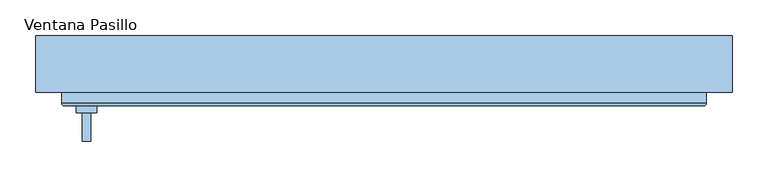
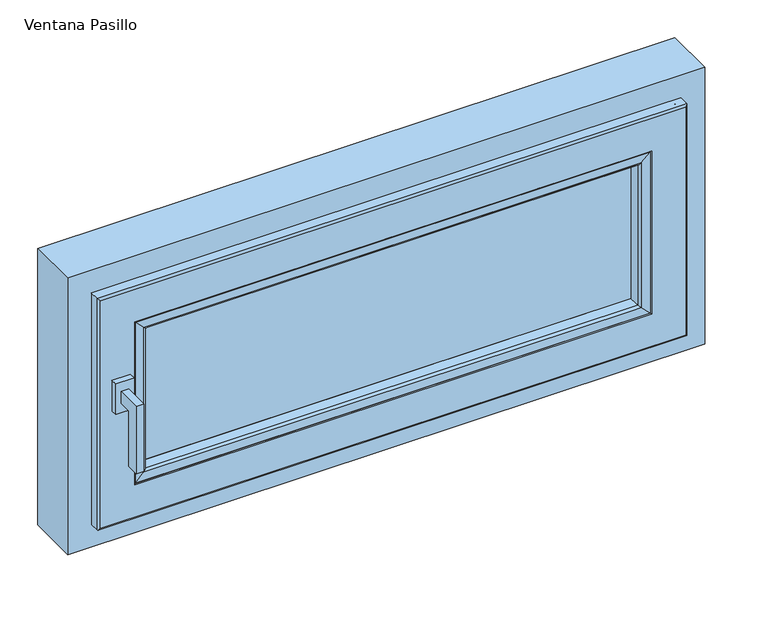
"""IFC4 building model written with IfcOpenShell, lengths in millimetres: window geometry, 2019_ES_Ventana_Replus_re80pvc301_10100_1-Hoja : Ventana Pasillo."""

import ifcopenshell
import ifcopenshell.guid

model = None  # the IFC model being written
_history = None  # IfcOwnerHistory: only IFC2X3 demands one
_inside = {}  # id of a spatial element -> (the spatial element, [elements in it])
_under = {}  # id of a project, library or spatial element -> (it, [spatial elements below it])
_declared = {}  # id of a project -> (the project, [libraries it declares])
_typed = {}  # id of a type object -> (the type object, [elements of that type])
_made_of = {}  # id of a material, layer set ... -> (it, [elements and type objects made of it])


def new_model(schema):
    """Start an empty IFC model of exactly this schema.

    Asked for "IFC4X3", IfcOpenShell would pick the latest addendum, in which some entities
    have other attributes; the version numbers below select the first issue.
    IFC2X3 requires an IfcOwnerHistory on every rooted entity: one is made here for all.
    """
    global model, _history
    if schema == "IFC4X3":
        model = ifcopenshell.file(schema_version=(4, 3, 0, 0))
    else:
        model = ifcopenshell.file(schema=schema)
    _inside.clear()
    _under.clear()
    _declared.clear()
    _typed.clear()
    _made_of.clear()
    _history = None
    if model.schema == "IFC2X3":
        org = make("IfcOrganization", Name="unknown")
        user = make(
            "IfcPersonAndOrganization",
            ThePerson=make("IfcPerson", FamilyName="unknown"),
            TheOrganization=org,
        )
        app = make(
            "IfcApplication",
            ApplicationDeveloper=org,
            Version="unknown",
            ApplicationFullName="unknown",
            ApplicationIdentifier="unknown",
        )
        _history = make(
            "IfcOwnerHistory",
            OwningUser=user,
            OwningApplication=app,
            ChangeAction="ADDED",
            CreationDate=0,
        )
    return model


def make(cls, **values):
    """One entity of the class cls with the attributes given. An attribute that is None is left unset."""
    return model.create_entity(
        cls, **{name: value for name, value in values.items() if value is not None}
    )


def rooted(cls, **values):
    """An entity with a GlobalId (a new one), such as an element, a storey or a relation."""
    return make(cls, GlobalId=ifcopenshell.guid.new(), OwnerHistory=_history, **values)


def si_unit(unit_type, name, prefix=None):
    """IfcSIUnit, for example si_unit("LENGTHUNIT", "METRE", prefix="MILLI")."""
    return make("IfcSIUnit", UnitType=unit_type, Prefix=prefix, Name=name)


def assignment(units):
    """IfcUnitAssignment: the units of a project."""
    return None if units is None else make("IfcUnitAssignment", Units=units)


def point(xyz):
    """IfcCartesianPoint."""
    return None if xyz is None else make("IfcCartesianPoint", Coordinates=xyz)


def direction(xyz):
    """IfcDirection."""
    return None if xyz is None else make("IfcDirection", DirectionRatios=xyz)


def frame(location, z_axis=None, x_axis=None):
    """IfcAxis2Placement3D, a coordinate frame: its origin and axes. An axis left out is left unset."""
    return make(
        "IfcAxis2Placement3D",
        Location=point(location),
        Axis=direction(z_axis),
        RefDirection=direction(x_axis),
    )


def origin():
    """The frame at (0, 0, 0) with its axes left unset."""
    return frame((0.0, 0.0, 0.0))


def place(relative_to, where):
    """IfcLocalPlacement: puts the frame where relative to a parent placement (None: the world)."""
    return make(
        "IfcLocalPlacement", PlacementRelTo=relative_to, RelativePlacement=where
    )


def context(
    kind, dimensions, precision=None, world=None, true_north=None, identifier=None
):
    """IfcGeometricRepresentationContext, for example the 3D "Model" context."""
    return make(
        "IfcGeometricRepresentationContext",
        ContextIdentifier=identifier,
        ContextType=kind,
        CoordinateSpaceDimension=dimensions,
        Precision=precision,
        WorldCoordinateSystem=world,
        TrueNorth=true_north,
    )


def project(units=None, contexts=None):
    """IfcProject with its units and contexts."""
    return rooted(
        "IfcProject",
        Name="project",
        RepresentationContexts=contexts,
        UnitsInContext=assignment(units),
    )


def spatial(cls, under=None, at=None, **own):
    """A site, building, storey or space (cls), placed at a placement, below another one or the project."""
    s = rooted(cls, ObjectPlacement=at, **own)
    if under is not None:
        _under.setdefault(under.id(), (under, []))[1].append(s)
    return s


def polyline(points):
    """IfcPolyline through the points."""
    return make("IfcPolyline", Points=[point(p) for p in points])


def ellipse_curve(where, semi_axis1, semi_axis2):
    """IfcEllipse in the frame where."""
    return make(
        "IfcEllipse", Position=where, SemiAxis1=semi_axis1, SemiAxis2=semi_axis2
    )


def outline(outer, holes=None, kind="AREA"):
    """IfcArbitraryClosedProfileDef: a profile drawn as a closed curve; with holes, ...WithVoids."""
    if holes is None:
        return make("IfcArbitraryClosedProfileDef", ProfileType=kind, OuterCurve=outer)
    return make(
        "IfcArbitraryProfileDefWithVoids",
        ProfileType=kind,
        OuterCurve=outer,
        InnerCurves=holes,
    )


def extrude(swept, where, along, depth):
    """IfcExtrudedAreaSolid: the profile swept, set in the frame where, extruded along a direction by depth."""
    return make(
        "IfcExtrudedAreaSolid",
        SweptArea=swept,
        Position=where,
        ExtrudedDirection=direction(along),
        Depth=depth,
    )


def shape(context_of_items, identifier, shape_type, items):
    """IfcShapeRepresentation: the items that make up one representation, for example the "Body"."""
    return make(
        "IfcShapeRepresentation",
        ContextOfItems=context_of_items,
        RepresentationIdentifier=identifier,
        RepresentationType=shape_type,
        Items=items,
    )


def source(mapping_origin, context_of_items, identifier, shape_type, items):
    """IfcRepresentationMap: a shape defined once, which mapped items show again and again."""
    return make(
        "IfcRepresentationMap",
        MappingOrigin=mapping_origin,
        MappedRepresentation=shape(context_of_items, identifier, shape_type, items),
    )


def transform(
    local_origin,
    x_axis=None,
    y_axis=None,
    z_axis=None,
    scale=None,
    scale2=None,
    scale3=None,
    uniform=True,
):
    """IfcCartesianTransformationOperator3D, or its non-uniform kind. x_axis, y_axis, z_axis: its Axis1, 2, 3."""
    if uniform:
        return make(
            "IfcCartesianTransformationOperator3D",
            Axis1=direction(x_axis),
            Axis2=direction(y_axis),
            LocalOrigin=point(local_origin),
            Scale=scale,
            Axis3=direction(z_axis),
        )
    return make(
        "IfcCartesianTransformationOperator3DnonUniform",
        Axis1=direction(x_axis),
        Axis2=direction(y_axis),
        LocalOrigin=point(local_origin),
        Scale=scale,
        Axis3=direction(z_axis),
        Scale2=scale2,
        Scale3=scale3,
    )


def mapped(mapping_source, mapping_target):
    """IfcMappedItem: shows the shape of a source again, moved by a transform."""
    return make(
        "IfcMappedItem", MappingSource=mapping_source, MappingTarget=mapping_target
    )


def made_of(thing, what):
    """Note that an element or type object is made of a material, layer set ...; save() writes the relation."""
    if what is not None:
        _made_of.setdefault(what.id(), (what, []))[1].append(thing)
    return thing


def element(
    cls,
    number,
    at=None,
    inside=None,
    cuts=None,
    type_object=None,
    material=None,
    context=None,
    identifier="Body",
    shape_type=None,
    held_by="IfcProductDefinitionShape",
    body=None,
    shapes=None,
    **own,
):
    """One element of the class cls, such as IfcWall. Its Tag is "e" and its number.

    at: its placement. inside: the storey or other place that contains it. cuts: it is an
    opening in that element (IfcRelVoidsElement). A single representation is given by context,
    identifier, shape_type and body (its items); several are given by shapes. held_by: the class
    of the entity that holds the representations. save() writes the other relations.
    """
    e = rooted(cls, Tag="e%d" % number, ObjectPlacement=at, **own)
    if body is not None:
        shapes = [shape(context, identifier, shape_type, body)]
    if shapes is not None:
        e.Representation = make(held_by, Representations=shapes)
    if inside is not None:
        _inside.setdefault(inside.id(), (inside, []))[1].append(e)
    if cuts is not None:
        rooted(
            "IfcRelVoidsElement", RelatingBuildingElement=cuts, RelatedOpeningElement=e
        )
    if type_object is not None:
        _typed.setdefault(type_object.id(), (type_object, []))[1].append(e)
    return made_of(e, material)


def aggregate(whole, parts):
    """IfcRelAggregates: a whole, such as a stair, and the parts it consists of."""
    return rooted("IfcRelAggregates", RelatingObject=whole, RelatedObjects=parts)


def save(model, path):
    """Write the relations noted so far, then the file.

    IfcRelAggregates (storeys below a building ...), IfcRelContainedInSpatialStructure (elements
    in a storey), IfcRelDefinesByType, IfcRelAssociatesMaterial and IfcRelDeclares: one each for
    every whole, place, type object, material and project.
    """
    for whole, parts in _under.values():
        aggregate(whole, parts)
    for where, things in _inside.values():
        rooted(
            "IfcRelContainedInSpatialStructure",
            RelatedElements=things,
            RelatingStructure=where,
        )
    for kind, things in _typed.values():
        rooted("IfcRelDefinesByType", RelatedObjects=things, RelatingType=kind)
    for what, things in _made_of.values():
        rooted("IfcRelAssociatesMaterial", RelatedObjects=things, RelatingMaterial=what)
    for by, libraries in _declared.values():
        rooted("IfcRelDeclares", RelatingContext=by, RelatedDefinitions=libraries)
    model.write(path)


def plane_surface(at):
    """IfcPlane: the flat surface through the origin of the frame at, square to its z axis."""
    return make("IfcPlane", Position=at)


def cylinder_surface(at, radius):
    """IfcCylindricalSurface: all points at the distance radius from the z axis of the frame at."""
    return make("IfcCylindricalSurface", Position=at, Radius=radius)


def advanced_brep(points, edges, surfaces, faces):
    """IfcAdvancedBrep: a solid bounded by faces that lie on surfaces and meet in shared edges.

    An edge is (start, end): straight between two places in points (the first is 0);
    or (start, end, curve); or (start, end, curve, False) where it runs against its curve.
    A face is (place in surfaces, loops), or (place, loops, False) where it looks against
    its surface's normal. A loop lists edges by number (the first is 1), with a minus sign
    where the edge is run from its end to its start. The first loop is the outer one.
    """
    corners = [point(p) for p in points]
    vertices = [make("IfcVertexPoint", VertexGeometry=c) for c in corners]
    made = []
    for start, end, *more in edges:
        made.append(
            make(
                "IfcEdgeCurve",
                EdgeStart=vertices[start],
                EdgeEnd=vertices[end],
                EdgeGeometry=more[0] if more else make("IfcPolyline", Points=[corners[start], corners[end]]),
                SameSense=more[1] if len(more) > 1 else True,
            )
        )
    hull = []
    for where, loops, *sense in faces:
        bounds = []
        for j, loop in enumerate(loops):
            ring = [make("IfcOrientedEdge", EdgeElement=made[abs(k) - 1], Orientation=k > 0) for k in loop]
            bounds.append(
                make(
                    "IfcFaceOuterBound" if j == 0 else "IfcFaceBound",
                    Bound=make("IfcEdgeLoop", EdgeList=ring),
                    Orientation=True,
                )
            )
        hull.append(make("IfcAdvancedFace", Bounds=bounds, FaceSurface=surfaces[where], SameSense=sense[0] if sense else True))
    return make("IfcAdvancedBrep", Outer=make("IfcClosedShell", CfsFaces=hull))


def ventana_pasillo_7f72e0b0(model_context):
    return source(origin(), model_context, "Body", "SolidModel", [
        extrude(outline(polyline([(-78.4999991, 1070.0), (-78.4999991, 1050.0), (-98.4999991, 1050.0), (-98.4999991, 960.0), (-118.4999991, 960.0), (-118.4999991, 1070.0), (-78.4999991, 1070.0)])), frame((-424.1999993, 0.0, 0.0), z_axis=(1.0, 0.0, 0.0), x_axis=(0.0, 1.0, 0.0)), (0.0, 0.0, 1.0), 12.0),
        extrude(outline(polyline([(-403.9687607, -78.4999991), (-432.4312378, -78.4999991), (-432.4312378, -68.4999991), (-403.9687607, -68.4999991), (-403.9687607, -78.4999991)])), frame((0.0, 0.0, 1035.217127), z_axis=(0.0, 0.0, 1.0), x_axis=(1.0, 0.0, 0.0)), (0.0, 0.0, 1.0), 49.565746),
        extrude(outline(polyline([(1157.2, 387.1999993), (1157.2, -387.1999993), (909.8, -387.1999993), (909.8, 387.1999993), (1157.2, 387.1999993)]), holes=[polyline([(917.8, 379.1999993), (917.8, -379.1999993), (1149.2, -379.1999993), (1149.2, 379.1999993), (917.8, 379.1999993)])]), frame((0.0, -26.9999999, 0.0), z_axis=(0.0, 1.0, 0.0), x_axis=(0.0, 0.0, 1.0)), (0.0, 0.0, 1.0), 16.0),
        extrude(outline(polyline([(1157.1868066, 387.1868058), (1157.1868066, -387.1868058), (909.8131934, -387.1868058), (909.8131934, 387.1868058), (1157.1868066, 387.1868058)]), holes=[polyline([(917.8, 379.1999993), (917.8, -379.1999993), (1149.2, -379.1999993), (1149.2, 379.1999993), (917.8, 379.1999993)])]), frame((0.0, -47.0000001, 0.0), z_axis=(0.0, 1.0, 0.0), x_axis=(0.0, 0.0, 1.0)), (0.0, 0.0, 1.0), 16.0),
        extrude(outline(polyline([(387.1999993, -6.9999997), (387.1999993, -10.9999999), (-387.1999993, -10.9999999), (-387.1999993, -6.9999997), (387.1999993, -6.9999997)])), frame((0.0, 0.0, 903.7946451), z_axis=(0.0, 0.0, 1.0), x_axis=(1.0, 0.0, 0.0)), (0.0, 0.0, 1.0), 259.4053549),
        extrude(outline(polyline([(387.1999993, -26.9999999), (387.1999993, -31.0000001), (-387.1999993, -31.0000001), (-387.1999993, -26.9999999), (387.1999993, -26.9999999)])), frame((0.0, 0.0, 903.7946451), z_axis=(0.0, 0.0, 1.0), x_axis=(1.0, 0.0, 0.0)), (0.0, 0.0, 1.0), 259.4053549),
        extrude(outline(polyline([(387.1999993, -47.0000001), (387.1999993, -51.0000003), (-387.1999993, -51.0000003), (-387.1999993, -47.0000001), (387.1999993, -47.0000001)])), frame((0.0, 0.0, 903.7946451), z_axis=(0.0, 0.0, 1.0), x_axis=(1.0, 0.0, 0.0)), (0.0, 0.0, 1.0), 259.4053549),
        advanced_brep(
        [(377.2913171, 9.2764571, 1147.2913178), (380.1890946, 11.5, 1150.1890953), (380.1890946, 11.5, 919.8109047), (377.2913171, 9.2764571, 922.7086822), (420.1999993, 11.5, 879.8), (-420.1999993, 11.5, 879.8), (-420.1999993, 11.5, 1190.2), (420.1999993, 11.5, 1190.2), (-380.1890946, 11.5, 1150.1890953), (-380.1890946, 11.5, 919.8109047), (-377.2913171, 9.2764571, 922.7086822), (374.1757968, -2.3508228, 1144.1757976), (374.1757968, -2.3508228, 925.8242024), (-374.1757968, -2.3508228, 925.8242024), (374.6739305, -3.0000033, 1144.6739313), (374.6739305, -3.0000033, 925.3260687), (-374.6739305, -3.0000033, 925.3260687), (381.1999993, -3.0000033, 1151.2), (-381.1999993, -3.0000033, 1151.2), (-381.1999993, -3.0000033, 918.8), (381.1999993, -3.0000033, 918.8), (-374.6739305, -3.0000033, 1144.6739313), (381.1999993, -6.9999997, 1151.2), (381.1999993, -6.9999997, 918.8), (-381.1999993, -6.9999997, 918.8), (401.8162192, -6.9999997, 1171.8162199), (-401.8162192, -6.9999997, 1171.8162199), (-401.8162192, -6.9999997, 898.1837801), (401.8162192, -6.9999997, 898.1837801), (-381.1999993, -6.9999997, 1151.2), (399.1999993, -25.6153717, 1169.2), (399.1999993, -25.6153717, 900.8), (-399.1999993, -25.6153717, 900.8), (399.1999993, -56.4999995, 1169.2), (399.1999993, -56.4999995, 900.8), (-399.1999993, -56.4999995, 900.8), (-399.1999993, -56.4999995, 1169.2), (387.1999993, -56.4999995, 1157.2), (-387.1999993, -56.4999995, 1157.2), (-387.1999993, -56.4999995, 912.8), (387.1999993, -56.4999995, 912.8), (387.1999993, -51.0000003, 1157.2), (387.1999993, -51.0000003, 912.8), (-387.1999993, -51.0000003, 912.8), (-387.1999993, -51.0000003, 1157.2), (376.007687, -51.0000003, 1146.0076877), (-376.007687, -51.0000003, 1146.0076877), (-376.007687, -51.0000003, 923.9923123), (376.007687, -51.0000003, 923.9923123), (375.4940999, -51.6693201, 1145.4941006), (375.4940999, -51.6693201, 924.5058994), (-375.4940999, -51.6693201, 924.5058994), (378.8993918, -64.3780426, 1148.8993925), (378.8993918, -64.3780426, 921.1006075), (-378.8993918, -64.3780426, 921.1006075), (382.6234971, -67.3403297, 1152.6234978), (382.6234971, -67.3403297, 917.3765022), (-382.6234971, -67.3403297, 917.3765022), (395.6488427, -67.7951848, 1165.6488434), (395.6488427, -67.7951848, 904.3511566), (-395.6488427, -67.7951848, 904.3511566), (396.1999993, -67.2629391, 1166.2), (396.1999993, -67.2629391, 903.8), (-396.1999993, -67.2629391, 903.8), (397.4370593, -68.4999991, 1167.43706), (397.4370593, -68.4999991, 902.56294), (-397.4370593, -68.4999991, 902.56294), (450.1999993, -68.4999991, 1220.2), (-450.1999993, -68.4999991, 1220.2), (-450.1999993, -68.4999991, 849.8), (450.1999993, -68.4999991, 849.8), (-397.4370593, -68.4999991, 1167.43706), (453.1999993, -65.4999991, 1223.2), (453.1999993, -65.4999991, 846.8), (-453.1999993, -65.4999991, 846.8), (453.1999993, -50.0, 1223.2), (453.1999993, -50.0, 846.8), (-453.1999993, -50.0, 846.8), (-453.1999993, -50.0, 1223.2), (433.1999993, -50.0, 1203.2), (-433.1999993, -50.0, 1203.2), (-433.1999993, -50.0, 866.8), (433.1999993, -50.0, 866.8), (433.1999993, -11.9999991, 866.8), (433.1999993, -11.9999991, 1203.2), (-433.1999993, -11.9999991, 866.8), (-433.1999993, -11.9999991, 1203.2), (420.1999993, -11.9999991, 1190.2), (-420.1999993, -11.9999991, 1190.2), (-420.1999993, -11.9999991, 879.8), (420.1999993, -11.9999991, 879.8), (-377.2913171, 9.2764571, 1147.2913178), (-374.1757968, -2.3508228, 1144.1757976), (-399.1999993, -25.6153717, 1169.2), (-375.4940999, -51.6693201, 1145.4941006), (-378.8993918, -64.3780426, 1148.8993925), (-382.6234971, -67.3403297, 1152.6234978), (-395.6488427, -67.7951848, 1165.6488434), (-396.1999993, -67.2629391, 1166.2), (-453.1999993, -65.4999991, 1223.2)],
        [
            (0, 1, ellipse_curve(frame((380.1890946, 8.5, 1150.1890953), z_axis=(0.7071067811865475, 0.0, -0.7071067811865475), x_axis=(0.7071067811865474, 0.0, 0.7071067811865476)), 4.2426407, 3.0)),
            (1, 2),
            (2, 3, ellipse_curve(frame((380.1890946, 8.5, 919.8109047), z_axis=(0.7071067811865475, 0.0, 0.7071067811865475), x_axis=(-0.7071067811865474, 0.0, 0.7071067811865476)), 4.2426407, 3.0)),
            (3, 0),
            (4, 5),
            (5, 6),
            (6, 7),
            (7, 4),
            (1, 8),
            (8, 9),
            (9, 2),
            (9, 10, ellipse_curve(frame((-380.1890946, 8.5, 919.8109047), z_axis=(0.7071067811865475, 0.0, -0.7071067811865475), x_axis=(0.7071067811865476, 0.0, 0.7071067811865474)), 4.2426407, 3.0)),
            (10, 3),
            (11, 0),
            (3, 12),
            (12, 11),
            (10, 13),
            (13, 12),
            (14, 11, ellipse_curve(frame((374.6739305, -2.4842973, 1144.6739313), z_axis=(0.7071067811865475, 0.0, -0.7071067811865475), x_axis=(0.7071067811865474, 0.0, 0.7071067811865476)), 0.7293184, 0.515706)),
            (12, 15, ellipse_curve(frame((374.6739305, -2.4842973, 925.3260687), z_axis=(0.7071067811865475, 0.0, 0.7071067811865475), x_axis=(-0.7071067811865474, 0.0, 0.7071067811865476)), 0.7293184, 0.515706)),
            (15, 14),
            (13, 16, ellipse_curve(frame((-374.6739305, -2.4842973, 925.3260687), z_axis=(0.7071067811865475, 0.0, -0.7071067811865475), x_axis=(0.7071067811865476, 0.0, 0.7071067811865474)), 0.7293184, 0.515706)),
            (16, 15),
            (17, 18),
            (18, 19),
            (19, 20),
            (20, 17),
            (16, 21),
            (21, 14),
            (22, 17),
            (20, 23),
            (23, 22),
            (19, 24),
            (24, 23),
            (25, 26),
            (26, 27),
            (27, 28),
            (28, 25),
            (24, 29),
            (29, 22),
            (30, 25),
            (28, 31),
            (31, 30),
            (27, 32),
            (32, 31),
            (33, 30),
            (31, 34),
            (34, 33),
            (32, 35),
            (35, 34),
            (35, 36),
            (36, 33),
            (37, 38),
            (38, 39),
            (39, 40),
            (40, 37),
            (41, 37),
            (40, 42),
            (42, 41),
            (39, 43),
            (43, 42),
            (43, 44),
            (44, 41),
            (45, 46),
            (46, 47),
            (47, 48),
            (48, 45),
            (49, 45, ellipse_curve(frame((376.007687, -51.5317048, 1146.0076877), z_axis=(0.7071067811865475, 0.0, -0.7071067811865475), x_axis=(0.7071067811865474, 0.0, 0.7071067811865476)), 0.7519437, 0.5317045)),
            (48, 50, ellipse_curve(frame((376.007687, -51.5317048, 923.9923123), z_axis=(0.7071067811865475, 0.0, 0.7071067811865475), x_axis=(-0.7071067811865474, 0.0, 0.7071067811865476)), 0.7519437, 0.5317045)),
            (50, 49),
            (47, 51, ellipse_curve(frame((-376.007687, -51.5317048, 923.9923123), z_axis=(0.7071067811865475, 0.0, -0.7071067811865475), x_axis=(0.7071067811865476, 0.0, 0.7071067811865474)), 0.7519437, 0.5317045)),
            (51, 50),
            (52, 49),
            (50, 53),
            (53, 52),
            (51, 54),
            (54, 53),
            (55, 52, ellipse_curve(frame((382.7630951, -63.3427664, 1152.7630958), z_axis=(0.7071067811865475, 0.0, -0.7071067811865475), x_axis=(0.7071067811865474, 0.0, 0.7071067811865476)), 5.6568542, 4.0)),
            (53, 56, ellipse_curve(frame((382.7630951, -63.3427664, 917.2369042), z_axis=(0.7071067811865475, 0.0, 0.7071067811865475), x_axis=(-0.7071067811865474, 0.0, 0.7071067811865476)), 5.6568542, 4.0)),
            (56, 55),
            (54, 57, ellipse_curve(frame((-382.7630951, -63.3427664, 917.2369042), z_axis=(0.7071067811865475, 0.0, -0.7071067811865475), x_axis=(0.7071067811865476, 0.0, 0.7071067811865474)), 5.6568542, 4.0)),
            (57, 56),
            (58, 55),
            (56, 59),
            (59, 58),
            (57, 60),
            (60, 59),
            (61, 58, ellipse_curve(frame((395.6674291, -67.2629391, 1165.6674299), z_axis=(0.7071067811865475, 0.0, -0.7071067811865475), x_axis=(0.7071067811865474, 0.0, 0.7071067811865476)), 0.7531679, 0.5325701)),
            (59, 62, ellipse_curve(frame((395.6674291, -67.2629391, 904.3325701), z_axis=(0.7071067811865475, 0.0, 0.7071067811865475), x_axis=(-0.7071067811865474, 0.0, 0.7071067811865476)), 0.7531679, 0.5325701)),
            (62, 61),
            (60, 63, ellipse_curve(frame((-395.6674291, -67.2629391, 904.3325701), z_axis=(0.7071067811865475, 0.0, -0.7071067811865475), x_axis=(0.7071067811865476, 0.0, 0.7071067811865474)), 0.7531679, 0.5325701)),
            (63, 62),
            (64, 61, ellipse_curve(frame((397.4370593, -67.2629391, 1167.43706), z_axis=(0.7071067811865475, 0.0, -0.7071067811865475), x_axis=(0.7071067811865474, 0.0, 0.7071067811865476)), 1.7494671, 1.23706)),
            (62, 65, ellipse_curve(frame((397.4370593, -67.2629391, 902.56294), z_axis=(0.7071067811865475, 0.0, 0.7071067811865475), x_axis=(-0.7071067811865474, 0.0, 0.7071067811865476)), 1.7494671, 1.23706)),
            (65, 64),
            (63, 66, ellipse_curve(frame((-397.4370593, -67.2629391, 902.56294), z_axis=(0.7071067811865475, 0.0, -0.7071067811865475), x_axis=(0.7071067811865476, 0.0, 0.7071067811865474)), 1.7494671, 1.23706)),
            (66, 65),
            (67, 68),
            (68, 69),
            (69, 70),
            (70, 67),
            (66, 71),
            (71, 64),
            (72, 67, ellipse_curve(frame((450.1999993, -65.4999991, 1220.2), z_axis=(0.7071067811865475, 0.0, -0.7071067811865475), x_axis=(0.7071067811865474, 0.0, 0.7071067811865476)), 4.2426407, 3.0)),
            (70, 73, ellipse_curve(frame((450.1999993, -65.4999991, 849.8), z_axis=(0.7071067811865475, 0.0, 0.7071067811865475), x_axis=(-0.7071067811865474, 0.0, 0.7071067811865476)), 4.2426407, 3.0)),
            (73, 72),
            (69, 74, ellipse_curve(frame((-450.1999993, -65.4999991, 849.8), z_axis=(0.7071067811865475, 0.0, -0.7071067811865475), x_axis=(0.7071067811865476, 0.0, 0.7071067811865474)), 4.2426407, 3.0)),
            (74, 73),
            (75, 72),
            (73, 76),
            (76, 75),
            (74, 77),
            (77, 76),
            (77, 78),
            (78, 75),
            (79, 80),
            (80, 81),
            (81, 82),
            (82, 79),
            (82, 83),
            (83, 84),
            (84, 79),
            (81, 85),
            (85, 83),
            (85, 86),
            (86, 84),
            (87, 88),
            (88, 89),
            (89, 90),
            (90, 87),
            (90, 4),
            (7, 87),
            (89, 5),
            (8, 91, ellipse_curve(frame((-380.1890946, 8.5, 1150.1890953), z_axis=(-0.7071067811865475, 0.0, -0.7071067811865475), x_axis=(0.7071067811865474, 0.0, -0.7071067811865476)), 4.2426407, 3.0)),
            (91, 10),
            (91, 92),
            (92, 13),
            (92, 21, ellipse_curve(frame((-374.6739305, -2.4842973, 1144.6739313), z_axis=(-0.7071067811865475, 0.0, -0.7071067811865475), x_axis=(0.7071067811865474, 0.0, -0.7071067811865476)), 0.7293184, 0.515706)),
            (18, 29),
            (26, 93),
            (93, 32),
            (93, 36),
            (38, 44),
            (46, 94, ellipse_curve(frame((-376.007687, -51.5317048, 1146.0076877), z_axis=(-0.7071067811865475, 0.0, -0.7071067811865475), x_axis=(0.7071067811865474, 0.0, -0.7071067811865476)), 0.7519437, 0.5317045)),
            (94, 51),
            (94, 95),
            (95, 54),
            (95, 96, ellipse_curve(frame((-382.7630951, -63.3427664, 1152.7630958), z_axis=(-0.7071067811865475, 0.0, -0.7071067811865475), x_axis=(0.7071067811865474, 0.0, -0.7071067811865476)), 5.6568542, 4.0)),
            (96, 57),
            (96, 97),
            (97, 60),
            (97, 98, ellipse_curve(frame((-395.6674291, -67.2629391, 1165.6674299), z_axis=(-0.7071067811865475, 0.0, -0.7071067811865475), x_axis=(0.7071067811865474, 0.0, -0.7071067811865476)), 0.7531679, 0.5325701)),
            (98, 63),
            (98, 71, ellipse_curve(frame((-397.4370593, -67.2629391, 1167.43706), z_axis=(-0.7071067811865475, 0.0, -0.7071067811865475), x_axis=(0.7071067811865474, 0.0, -0.7071067811865476)), 1.7494671, 1.23706)),
            (68, 99, ellipse_curve(frame((-450.1999993, -65.4999991, 1220.2), z_axis=(-0.7071067811865475, 0.0, -0.7071067811865475), x_axis=(0.7071067811865474, 0.0, -0.7071067811865476)), 4.2426407, 3.0)),
            (99, 74),
            (99, 78),
            (80, 86),
            (88, 6),
            (0, 91),
            (11, 92),
            (30, 93),
            (49, 94),
            (52, 95),
            (55, 96),
            (58, 97),
            (61, 98),
            (72, 99),
        ],
        [
            cylinder_surface(frame((380.1890946, 8.5, 1223.2), z_axis=(0.0, 0.0, 1.0), x_axis=(-1.0, 0.0, 0.0)), 3.0),
            plane_surface(frame((-420.1999993, 11.5, 1190.2), z_axis=(0.0, 1.0, 0.0), x_axis=(1.0, 0.0, 0.0))),
            cylinder_surface(frame((453.1999993, 8.5, 919.8109047), z_axis=(1.0, 0.0, 0.0), x_axis=(0.0, 0.0, 1.0)), 3.0),
            plane_surface(frame((377.2913171, 9.2764571, 1147.2913178), z_axis=(-0.9659258263570549, 0.25881904484879154, 0.0), x_axis=(0.0, 0.0, -1.0))),
            plane_surface(frame((377.2913171, 9.2764571, 922.7086822), z_axis=(0.0, 0.2588190448487884, 0.9659258263570558), x_axis=(-1.0, 0.0, 0.0))),
            cylinder_surface(frame((374.6739305, -2.4842973, 1223.2), z_axis=(0.0, 0.0, 1.0), x_axis=(-1.0, 0.0, 0.0)), 0.515706),
            cylinder_surface(frame((453.1999993, -2.4842973, 925.3260687), z_axis=(1.0, 0.0, 0.0), x_axis=(0.0, 0.0, 1.0)), 0.515706),
            plane_surface(frame((-374.6739305, -3.0000033, 1144.6739313), z_axis=(0.0, -1.0, 0.0), x_axis=(1.0, 0.0, 0.0))),
            plane_surface(frame((381.1999993, -3.0000033, 1151.2), z_axis=(-1.0, 0.0, 0.0), x_axis=(0.0, 0.0, -1.0))),
            plane_surface(frame((381.1999993, -3.0000033, 918.8), z_axis=(0.0, 0.0, 1.0), x_axis=(-1.0, 0.0, 0.0))),
            plane_surface(frame((-381.1999993, -6.9999997, 1151.2), z_axis=(0.0, -1.0, 0.0), x_axis=(1.0, 0.0, 0.0))),
            plane_surface(frame((401.8162192, -6.9999997, 1171.8162199), z_axis=(-0.9902680687415736, 0.13917310096004262, 0.0), x_axis=(0.0, 0.0, -1.0))),
            plane_surface(frame((401.8162192, -6.9999997, 898.1837801), z_axis=(0.0, 0.13917310096003943, 0.990268068741574), x_axis=(-1.0, 0.0, 0.0))),
            plane_surface(frame((399.1999993, -25.6153717, 1169.2), z_axis=(-1.0, 0.0, 0.0), x_axis=(0.0, 0.0, -1.0))),
            plane_surface(frame((399.1999993, -25.6153717, 900.8), z_axis=(0.0, 0.0, 1.0), x_axis=(-1.0, 0.0, 0.0))),
            plane_surface(frame((-399.1999993, -56.4999995, 1169.2), z_axis=(0.0, 1.0, 0.0), x_axis=(1.0, 0.0, 0.0))),
            plane_surface(frame((387.1999993, -56.4999995, 1157.2), z_axis=(1.0, 0.0, 0.0), x_axis=(0.0, 0.0, -1.0))),
            plane_surface(frame((387.1999993, -56.4999995, 912.8), z_axis=(0.0, 0.0, -1.0), x_axis=(-1.0, 0.0, 0.0))),
            plane_surface(frame((-387.1999993, -51.0000003, 1157.2), z_axis=(0.0, 1.0, 0.0), x_axis=(1.0, 0.0, 0.0))),
            cylinder_surface(frame((376.007687, -51.5317048, 1223.2), z_axis=(0.0, 0.0, 1.0), x_axis=(-1.0, 0.0, 0.0)), 0.5317045),
            cylinder_surface(frame((453.1999993, -51.5317048, 923.9923123), z_axis=(1.0, 0.0, 0.0), x_axis=(0.0, 0.0, 1.0)), 0.5317045),
            plane_surface(frame((375.4940999, -51.6693201, 1145.4941006), z_axis=(-0.9659258262890666, -0.25881904510252723, 0.0), x_axis=(0.0, 0.0, -1.0))),
            plane_surface(frame((375.4940999, -51.6693201, 924.5058994), z_axis=(0.0, -0.25881904510253034, 0.9659258262890658), x_axis=(-1.0, 0.0, 0.0))),
            cylinder_surface(frame((382.7630951, -63.3427664, 1223.2), z_axis=(0.0, 0.0, 1.0), x_axis=(-1.0, 0.0, 0.0)), 4.0),
            cylinder_surface(frame((453.1999993, -63.3427664, 917.2369042), z_axis=(1.0, 0.0, 0.0), x_axis=(0.0, 0.0, 1.0)), 4.0),
            plane_surface(frame((382.6234971, -67.3403297, 1152.6234978), z_axis=(-0.0348994967025078, -0.9993908270190955, 0.0), x_axis=(0.0, 0.0, -1.0))),
            plane_surface(frame((382.6234971, -67.3403297, 917.3765022), z_axis=(0.0, -0.9993908270190957, 0.03489949670250457), x_axis=(-1.0, 0.0, 0.0))),
            cylinder_surface(frame((395.6674291, -67.2629391, 1223.2), z_axis=(0.0, 0.0, 1.0), x_axis=(-1.0, 0.0, 0.0)), 0.5325701),
            cylinder_surface(frame((453.1999993, -67.2629391, 904.3325701), z_axis=(1.0, 0.0, 0.0), x_axis=(0.0, 0.0, 1.0)), 0.5325701),
            cylinder_surface(frame((397.4370593, -67.2629391, 1223.2), z_axis=(0.0, 0.0, 1.0), x_axis=(-1.0, 0.0, 0.0)), 1.23706),
            cylinder_surface(frame((453.1999993, -67.2629391, 902.56294), z_axis=(1.0, 0.0, 0.0), x_axis=(0.0, 0.0, 1.0)), 1.23706),
            plane_surface(frame((-397.4370593, -68.4999991, 1167.43706), z_axis=(0.0, -1.0, 0.0), x_axis=(1.0, 0.0, 0.0))),
            cylinder_surface(frame((450.1999993, -65.4999991, 1223.2), z_axis=(0.0, 0.0, 1.0), x_axis=(-1.0, 0.0, 0.0)), 3.0),
            cylinder_surface(frame((453.1999993, -65.4999991, 849.8), z_axis=(1.0, 0.0, 0.0), x_axis=(0.0, 0.0, 1.0)), 3.0),
            plane_surface(frame((453.1999993, -65.4999991, 1223.2), z_axis=(1.0, 0.0, 0.0), x_axis=(0.0, 0.0, -1.0))),
            plane_surface(frame((453.1999993, -65.4999991, 846.8), z_axis=(0.0, 0.0, -1.0), x_axis=(-1.0, 0.0, 0.0))),
            plane_surface(frame((-449.2000019, -50.0, 1219.2000027), z_axis=(0.0, 1.0, 0.0), x_axis=(1.0, 0.0, 0.0))),
            plane_surface(frame((433.1999993, -45.0999991, 1203.2), z_axis=(1.0, 0.0, 0.0), x_axis=(0.0, 0.0, -1.0))),
            plane_surface(frame((433.1999993, -45.0999991, 866.8), z_axis=(0.0, 0.0, -1.0), x_axis=(-1.0, 0.0, 0.0))),
            plane_surface(frame((-425.7000002, -11.9999991, 1195.7000009), z_axis=(0.0, 1.0, 0.0), x_axis=(1.0, 0.0, 0.0))),
            plane_surface(frame((420.1999993, -1.4999991, 1190.2), z_axis=(1.0, 0.0, 0.0), x_axis=(0.0, 0.0, -1.0))),
            plane_surface(frame((420.1999993, -1.4999991, 879.8), z_axis=(0.0, 0.0, -1.0), x_axis=(-1.0, 0.0, 0.0))),
            cylinder_surface(frame((-380.1890946, 8.5, 846.8), z_axis=(0.0, 0.0, -1.0), x_axis=(1.0, 0.0, 0.0)), 3.0),
            plane_surface(frame((-377.2913171, 9.2764571, 922.7086822), z_axis=(0.9659258263570565, 0.25881904484878526, 0.0), x_axis=(0.0, 0.0, 1.0))),
            cylinder_surface(frame((-374.6739305, -2.4842973, 846.8), z_axis=(0.0, 0.0, -1.0), x_axis=(1.0, 0.0, 0.0)), 0.515706),
            plane_surface(frame((-381.1999993, -3.0000033, 918.8), z_axis=(1.0, 0.0, 0.0), x_axis=(0.0, 0.0, 1.0))),
            plane_surface(frame((-401.8162192, -6.9999997, 898.1837801), z_axis=(0.9902680687415745, 0.13917310096003624, 0.0), x_axis=(0.0, 0.0, 1.0))),
            plane_surface(frame((-399.1999993, -25.6153717, 900.8), z_axis=(1.0, 0.0, 0.0), x_axis=(0.0, 0.0, 1.0))),
            plane_surface(frame((-387.1999993, -56.4999995, 912.8), z_axis=(-1.0, 0.0, 0.0), x_axis=(0.0, 0.0, 1.0))),
            cylinder_surface(frame((-376.007687, -51.5317048, 846.8), z_axis=(0.0, 0.0, -1.0), x_axis=(1.0, 0.0, 0.0)), 0.5317045),
            plane_surface(frame((-375.4940999, -51.6693201, 924.5058994), z_axis=(0.9659258262890649, -0.25881904510253345, 0.0), x_axis=(0.0, 0.0, 1.0))),
            cylinder_surface(frame((-382.7630951, -63.3427664, 846.8), z_axis=(0.0, 0.0, -1.0), x_axis=(1.0, 0.0, 0.0)), 4.0),
            plane_surface(frame((-382.6234971, -67.3403297, 917.3765022), z_axis=(0.034899496702501344, -0.9993908270190958, 0.0), x_axis=(0.0, 0.0, 1.0))),
            cylinder_surface(frame((-395.6674291, -67.2629391, 846.8), z_axis=(0.0, 0.0, -1.0), x_axis=(1.0, 0.0, 0.0)), 0.5325701),
            cylinder_surface(frame((-397.4370593, -67.2629391, 846.8), z_axis=(0.0, 0.0, -1.0), x_axis=(1.0, 0.0, 0.0)), 1.23706),
            cylinder_surface(frame((-450.1999993, -65.4999991, 846.8), z_axis=(0.0, 0.0, -1.0), x_axis=(1.0, 0.0, 0.0)), 3.0),
            plane_surface(frame((-453.1999993, -65.4999991, 846.8), z_axis=(-1.0, 0.0, 0.0), x_axis=(0.0, 0.0, 1.0))),
            plane_surface(frame((-433.1999993, -45.0999991, 866.8), z_axis=(-1.0, 0.0, 0.0), x_axis=(0.0, 0.0, 1.0))),
            plane_surface(frame((-420.1999993, -1.4999991, 879.8), z_axis=(-1.0, 0.0, 0.0), x_axis=(0.0, 0.0, 1.0))),
            cylinder_surface(frame((-453.1999993, 8.5, 1150.1890953), z_axis=(-1.0, 0.0, 0.0), x_axis=(0.0, 0.0, -1.0)), 3.0),
            plane_surface(frame((-377.2913171, 9.2764571, 1147.2913178), z_axis=(0.0, 0.2588190448487884, -0.9659258263570557), x_axis=(1.0, 0.0, 0.0))),
            cylinder_surface(frame((-453.1999993, -2.4842973, 1144.6739313), z_axis=(-1.0, 0.0, 0.0), x_axis=(0.0, 0.0, -1.0)), 0.515706),
            plane_surface(frame((-381.1999993, -3.0000033, 1151.2), z_axis=(0.0, 0.0, -1.0), x_axis=(1.0, 0.0, 0.0))),
            plane_surface(frame((-401.8162192, -6.9999997, 1171.8162199), z_axis=(0.0, 0.13917310096003943, -0.990268068741574), x_axis=(1.0, 0.0, 0.0))),
            plane_surface(frame((-399.1999993, -25.6153717, 1169.2), z_axis=(0.0, 0.0, -1.0), x_axis=(1.0, 0.0, 0.0))),
            plane_surface(frame((-387.1999993, -56.4999995, 1157.2), z_axis=(0.0, 0.0, 1.0), x_axis=(1.0, 0.0, 0.0))),
            cylinder_surface(frame((-453.1999993, -51.5317048, 1146.0076877), z_axis=(-1.0, 0.0, 0.0), x_axis=(0.0, 0.0, -1.0)), 0.5317045),
            plane_surface(frame((-375.4940999, -51.6693201, 1145.4941006), z_axis=(0.0, -0.25881904510253034, -0.9659258262890658), x_axis=(1.0, 0.0, 0.0))),
            cylinder_surface(frame((-453.1999993, -63.3427664, 1152.7630958), z_axis=(-1.0, 0.0, 0.0), x_axis=(0.0, 0.0, -1.0)), 4.0),
            plane_surface(frame((-382.6234971, -67.3403297, 1152.6234978), z_axis=(0.0, -0.9993908270190957, -0.03489949670250457), x_axis=(1.0, 0.0, 0.0))),
            cylinder_surface(frame((-453.1999993, -67.2629391, 1165.6674299), z_axis=(-1.0, 0.0, 0.0), x_axis=(0.0, 0.0, -1.0)), 0.5325701),
            cylinder_surface(frame((-453.1999993, -67.2629391, 1167.43706), z_axis=(-1.0, 0.0, 0.0), x_axis=(0.0, 0.0, -1.0)), 1.23706),
            cylinder_surface(frame((-453.1999993, -65.4999991, 1220.2), z_axis=(-1.0, 0.0, 0.0), x_axis=(0.0, 0.0, -1.0)), 3.0),
            plane_surface(frame((-453.1999993, -65.4999991, 1223.2), z_axis=(0.0, 0.0, 1.0), x_axis=(1.0, 0.0, 0.0))),
            plane_surface(frame((-433.1999993, -45.0999991, 1203.2), z_axis=(0.0, 0.0, 1.0), x_axis=(1.0, 0.0, 0.0))),
            plane_surface(frame((-420.1999993, -1.4999991, 1190.2), z_axis=(0.0, 0.0, 1.0), x_axis=(1.0, 0.0, 0.0))),
        ],
        [
            (0, [[1, 2, 3, 4]]),
            (1, [[5, 6, 7, 8], [9, 10, 11, -2]]),
            (2, [[-3, -11, 12, 13]]),
            (3, [[14, -4, 15, 16]]),
            (4, [[-15, -13, 17, 18]]),
            (5, [[19, -16, 20, 21]]),
            (6, [[-20, -18, 22, 23]]),
            (7, [[24, 25, 26, 27], [-23, 28, 29, -21]]),
            (8, [[30, -27, 31, 32]]),
            (9, [[-31, -26, 33, 34]]),
            (10, [[35, 36, 37, 38], [-34, 39, 40, -32]]),
            (11, [[41, -38, 42, 43]]),
            (12, [[-42, -37, 44, 45]]),
            (13, [[46, -43, 47, 48]]),
            (14, [[-47, -45, 49, 50]]),
            (15, [[-50, 51, 52, -48], [53, 54, 55, 56]]),
            (16, [[57, -56, 58, 59]]),
            (17, [[-58, -55, 60, 61]]),
            (18, [[-61, 62, 63, -59], [64, 65, 66, 67]]),
            (19, [[68, -67, 69, 70]]),
            (20, [[-69, -66, 71, 72]]),
            (21, [[73, -70, 74, 75]]),
            (22, [[-74, -72, 76, 77]]),
            (23, [[78, -75, 79, 80]]),
            (24, [[-79, -77, 81, 82]]),
            (25, [[83, -80, 84, 85]]),
            (26, [[-84, -82, 86, 87]]),
            (27, [[88, -85, 89, 90]]),
            (28, [[-89, -87, 91, 92]]),
            (29, [[93, -90, 94, 95]]),
            (30, [[-94, -92, 96, 97]]),
            (31, [[98, 99, 100, 101], [-97, 102, 103, -95]]),
            (32, [[104, -101, 105, 106]]),
            (33, [[-105, -100, 107, 108]]),
            (34, [[109, -106, 110, 111]]),
            (35, [[-110, -108, 112, 113]]),
            (36, [[-113, 114, 115, -111], [116, 117, 118, 119]]),
            (37, [[-119, 120, 121, 122]]),
            (38, [[-120, -118, 123, 124]]),
            (39, [[-124, 125, 126, -121], [127, 128, 129, 130]]),
            (40, [[-130, 131, -8, 132]]),
            (41, [[-131, -129, 133, -5]]),
            (42, [[-12, -10, 134, 135]]),
            (43, [[-17, -135, 136, 137]]),
            (44, [[-22, -137, 138, -28]]),
            (45, [[-33, -25, 139, -39]]),
            (46, [[-44, -36, 140, 141]]),
            (47, [[-49, -141, 142, -51]]),
            (48, [[-60, -54, 143, -62]]),
            (49, [[-71, -65, 144, 145]]),
            (50, [[-76, -145, 146, 147]]),
            (51, [[-81, -147, 148, 149]]),
            (52, [[-86, -149, 150, 151]]),
            (53, [[-91, -151, 152, 153]]),
            (54, [[-96, -153, 154, -102]]),
            (55, [[-107, -99, 155, 156]]),
            (56, [[-112, -156, 157, -114]]),
            (57, [[-123, -117, 158, -125]]),
            (58, [[-133, -128, 159, -6]]),
            (59, [[-134, -9, -1, 160]]),
            (60, [[-136, -160, -14, 161]]),
            (61, [[-138, -161, -19, -29]]),
            (62, [[-139, -24, -30, -40]]),
            (63, [[-140, -35, -41, 162]]),
            (64, [[-142, -162, -46, -52]]),
            (65, [[-143, -53, -57, -63]]),
            (66, [[-144, -64, -68, 163]]),
            (67, [[-146, -163, -73, 164]]),
            (68, [[-148, -164, -78, 165]]),
            (69, [[-150, -165, -83, 166]]),
            (70, [[-152, -166, -88, 167]]),
            (71, [[-154, -167, -93, -103]]),
            (72, [[-155, -98, -104, 168]]),
            (73, [[-157, -168, -109, -115]]),
            (74, [[-158, -116, -122, -126]]),
            (75, [[-159, -127, -132, -7]]),
        ],
    ),
        advanced_brep(
        [(413.2673545, 12.758819, 1183.2673545), (417.2913185, 27.7764571, 1187.2913185), (417.2913185, 27.7764571, 882.7086815), (413.2673545, 12.758819, 886.7326455), (420.189096, 30.0, 1190.189096), (420.189096, 30.0, 879.810904), (-417.2913185, 27.7764571, 882.7086815), (-413.2673545, 12.758819, 886.7326455), (414.2332803, 11.5, 1184.2332803), (414.2332803, 11.5, 885.7667197), (490.0, 30.0, 1260.0), (490.0, -50.0, 1260.0), (490.0, -50.0, 810.0), (490.0, 30.0, 810.0), (-490.0, -50.0, 1260.0), (-490.0, -50.0, 810.0), (446.1999993, -50.0, 853.8000007), (-446.1999993, -50.0, 853.8000007), (-446.1999993, -50.0, 1216.1999993), (446.1999993, -50.0, 1216.1999993), (-490.0, 30.0, 810.0), (-490.0, 30.0, 1260.0), (-420.189096, 30.0, 1190.189096), (-420.189096, 30.0, 879.810904), (426.1891471, -8.0, 1196.1891471), (426.1891471, 11.5, 1196.1891471), (426.1891471, 11.5, 873.8108529), (426.1891471, -8.0, 873.8108529), (-426.1891471, 11.5, 1196.1891471), (-426.1891471, 11.5, 873.8108529), (-414.2332803, 11.5, 885.7667197), (-414.2332803, 11.5, 1184.2332803), (-426.1891471, -8.0, 873.8108529), (445.1999993, -8.0, 1215.1999993), (-445.1999993, -8.0, 1215.1999993), (-445.1999993, -8.0, 854.8000007), (445.1999993, -8.0, 854.8000007), (-426.1891471, -8.0, 1196.1891471), (445.1999993, -49.0, 1215.1999993), (445.1999993, -49.0, 854.8000007), (-445.1999993, -49.0, 854.8000007), (-417.2913185, 27.7764571, 1187.2913185), (-413.2673545, 12.758819, 1183.2673545), (-445.1999993, -49.0, 1215.1999993)],
        [
            (0, 1),
            (1, 2),
            (2, 3),
            (3, 0),
            (1, 4, ellipse_curve(frame((420.189096, 27.0, 1190.189096), z_axis=(0.7071067811865475, 0.0, -0.7071067811865475), x_axis=(0.7071067811865474, 0.0, 0.7071067811865476)), 4.2426407, 3.0)),
            (4, 5),
            (5, 2, ellipse_curve(frame((420.189096, 27.0, 879.810904), z_axis=(0.7071067811865475, 0.0, 0.7071067811865475), x_axis=(-0.7071067811865474, 0.0, 0.7071067811865476)), 4.2426407, 3.0)),
            (2, 6),
            (6, 7),
            (7, 3),
            (8, 0, ellipse_curve(frame((414.2332803, 12.5, 1184.2332803), z_axis=(0.7071067811865475, 0.0, -0.7071067811865475), x_axis=(0.7071067811865474, 0.0, 0.7071067811865476)), 1.4142136, 1.0)),
            (3, 9, ellipse_curve(frame((414.2332803, 12.5, 885.7667197), z_axis=(0.7071067811865475, 0.0, 0.7071067811865475), x_axis=(-0.7071067811865474, 0.0, 0.7071067811865476)), 1.4142136, 1.0)),
            (9, 8),
            (10, 11),
            (11, 12),
            (12, 13),
            (13, 10),
            (11, 14),
            (14, 15),
            (15, 12),
            (16, 17),
            (17, 18),
            (18, 19),
            (19, 16),
            (15, 20),
            (20, 13),
            (20, 21),
            (21, 10),
            (4, 22),
            (22, 23),
            (23, 5),
            (24, 25),
            (25, 26),
            (26, 27),
            (27, 24),
            (25, 28),
            (28, 29),
            (29, 26),
            (9, 30),
            (30, 31),
            (31, 8),
            (29, 32),
            (32, 27),
            (33, 34),
            (34, 35),
            (35, 36),
            (36, 33),
            (32, 37),
            (37, 24),
            (19, 38, ellipse_curve(frame((446.1999993, -49.0, 1216.1999993), z_axis=(0.7071067811865475, 0.0, -0.7071067811865475), x_axis=(0.7071067811865474, 0.0, 0.7071067811865476)), 1.4142136, 1.0)),
            (38, 39),
            (39, 16, ellipse_curve(frame((446.1999993, -49.0, 853.8000007), z_axis=(0.7071067811865475, 0.0, 0.7071067811865475), x_axis=(-0.7071067811865474, 0.0, 0.7071067811865476)), 1.4142136, 1.0)),
            (38, 33),
            (36, 39),
            (39, 40),
            (40, 17, ellipse_curve(frame((-446.1999993, -49.0, 853.8000007), z_axis=(0.7071067811865475, 0.0, -0.7071067811865475), x_axis=(0.7071067811865476, 0.0, 0.7071067811865474)), 1.4142136, 1.0)),
            (7, 30, ellipse_curve(frame((-414.2332803, 12.5, 885.7667197), z_axis=(0.7071067811865475, 0.0, -0.7071067811865475), x_axis=(0.7071067811865476, 0.0, 0.7071067811865474)), 1.4142136, 1.0)),
            (23, 6, ellipse_curve(frame((-420.189096, 27.0, 879.810904), z_axis=(0.7071067811865475, 0.0, -0.7071067811865475), x_axis=(0.7071067811865476, 0.0, 0.7071067811865474)), 4.2426407, 3.0)),
            (6, 41),
            (41, 42),
            (42, 7),
            (14, 21),
            (28, 37),
            (35, 40),
            (40, 43),
            (43, 18, ellipse_curve(frame((-446.1999993, -49.0, 1216.1999993), z_axis=(-0.7071067811865475, 0.0, -0.7071067811865475), x_axis=(0.7071067811865474, 0.0, -0.7071067811865476)), 1.4142136, 1.0)),
            (42, 31, ellipse_curve(frame((-414.2332803, 12.5, 1184.2332803), z_axis=(-0.7071067811865475, 0.0, -0.7071067811865475), x_axis=(0.7071067811865474, 0.0, -0.7071067811865476)), 1.4142136, 1.0)),
            (22, 41, ellipse_curve(frame((-420.189096, 27.0, 1190.189096), z_axis=(-0.7071067811865475, 0.0, -0.7071067811865475), x_axis=(0.7071067811865474, 0.0, -0.7071067811865476)), 4.2426407, 3.0)),
            (34, 43),
            (41, 1),
            (0, 42),
            (43, 38),
        ],
        [
            plane_surface(frame((417.2913185, 27.7764571, 1187.2913185), z_axis=(-0.9659258262890693, 0.2588190451025169, 0.0), x_axis=(0.0, 0.0, -1.0))),
            cylinder_surface(frame((420.189096, 27.0, 1260.0), z_axis=(0.0, 0.0, 1.0), x_axis=(-1.0, 0.0, 0.0)), 3.0),
            plane_surface(frame((417.2913185, 27.7764571, 882.7086815), z_axis=(0.0, 0.2588190451025138, 0.9659258262890702), x_axis=(-1.0, 0.0, 0.0))),
            cylinder_surface(frame((414.2332803, 12.5, 1260.0), z_axis=(0.0, 0.0, 1.0), x_axis=(-1.0, 0.0, 0.0)), 1.0),
            plane_surface(frame((490.0, -50.0, 1260.0), z_axis=(1.0, 0.0, 0.0), x_axis=(0.0, 0.0, -1.0))),
            plane_surface(frame((-446.1999993, -50.0, 1216.1999993), z_axis=(0.0, -1.0, 0.0), x_axis=(1.0, 0.0, 0.0))),
            plane_surface(frame((490.0, -50.0, 810.0), z_axis=(0.0, 0.0, -1.0), x_axis=(-1.0, 0.0, 0.0))),
            plane_surface(frame((-490.0, 30.0, 1260.0), z_axis=(0.0, 1.0, 0.0), x_axis=(1.0, 0.0, 0.0))),
            plane_surface(frame((426.1891471, 11.5, 1196.1891471), z_axis=(-1.0, 0.0, 0.0), x_axis=(0.0, 0.0, -1.0))),
            plane_surface(frame((-414.2332803, 11.5, 1184.2332803), z_axis=(0.0, -1.0, 0.0), x_axis=(1.0, 0.0, 0.0))),
            plane_surface(frame((426.1891471, 11.5, 873.8108529), z_axis=(0.0, 0.0, 1.0), x_axis=(-1.0, 0.0, 0.0))),
            plane_surface(frame((-426.1891471, -8.0, 1196.1891471), z_axis=(0.0, -1.0, 0.0), x_axis=(1.0, 0.0, 0.0))),
            cylinder_surface(frame((446.1999993, -49.0, 1260.0), z_axis=(0.0, 0.0, 1.0), x_axis=(-1.0, 0.0, 0.0)), 1.0),
            plane_surface(frame((445.1999993, -8.0, 1215.1999993), z_axis=(-1.0, 0.0, 0.0), x_axis=(0.0, 0.0, -1.0))),
            cylinder_surface(frame((490.0, -49.0, 853.8000007), z_axis=(1.0, 0.0, 0.0), x_axis=(0.0, 0.0, 1.0)), 1.0),
            cylinder_surface(frame((490.0, 12.5, 885.7667197), z_axis=(1.0, 0.0, 0.0), x_axis=(0.0, 0.0, 1.0)), 1.0),
            cylinder_surface(frame((490.0, 27.0, 879.810904), z_axis=(1.0, 0.0, 0.0), x_axis=(0.0, 0.0, 1.0)), 3.0),
            plane_surface(frame((-417.2913185, 27.7764571, 882.7086815), z_axis=(0.9659258262890711, 0.2588190451025107, 0.0), x_axis=(0.0, 0.0, 1.0))),
            plane_surface(frame((-490.0, -50.0, 810.0), z_axis=(-1.0, 0.0, 0.0), x_axis=(0.0, 0.0, 1.0))),
            plane_surface(frame((-426.1891471, 11.5, 873.8108529), z_axis=(1.0, 0.0, 0.0), x_axis=(0.0, 0.0, 1.0))),
            plane_surface(frame((445.1999993, -8.0, 854.8000007), z_axis=(0.0, 0.0, 1.0), x_axis=(-1.0, 0.0, 0.0))),
            cylinder_surface(frame((-446.1999993, -49.0, 810.0), z_axis=(0.0, 0.0, -1.0), x_axis=(1.0, 0.0, 0.0)), 1.0),
            cylinder_surface(frame((-414.2332803, 12.5, 810.0), z_axis=(0.0, 0.0, -1.0), x_axis=(1.0, 0.0, 0.0)), 1.0),
            cylinder_surface(frame((-420.189096, 27.0, 810.0), z_axis=(0.0, 0.0, -1.0), x_axis=(1.0, 0.0, 0.0)), 3.0),
            plane_surface(frame((-445.1999993, -8.0, 854.8000007), z_axis=(1.0, 0.0, 0.0), x_axis=(0.0, 0.0, 1.0))),
            plane_surface(frame((-417.2913185, 27.7764571, 1187.2913185), z_axis=(0.0, 0.2588190451025138, -0.9659258262890702), x_axis=(1.0, 0.0, 0.0))),
            plane_surface(frame((-490.0, -50.0, 1260.0), z_axis=(0.0, 0.0, 1.0), x_axis=(1.0, 0.0, 0.0))),
            plane_surface(frame((-426.1891471, 11.5, 1196.1891471), z_axis=(0.0, 0.0, -1.0), x_axis=(1.0, 0.0, 0.0))),
            cylinder_surface(frame((-490.0, -49.0, 1216.1999993), z_axis=(-1.0, 0.0, 0.0), x_axis=(0.0, 0.0, -1.0)), 1.0),
            cylinder_surface(frame((-490.0, 12.5, 1184.2332803), z_axis=(-1.0, 0.0, 0.0), x_axis=(0.0, 0.0, -1.0)), 1.0),
            cylinder_surface(frame((-490.0, 27.0, 1190.189096), z_axis=(-1.0, 0.0, 0.0), x_axis=(0.0, 0.0, -1.0)), 3.0),
            plane_surface(frame((-445.1999993, -8.0, 1215.1999993), z_axis=(0.0, 0.0, -1.0), x_axis=(1.0, 0.0, 0.0))),
        ],
        [
            (0, [[1, 2, 3, 4]]),
            (1, [[5, 6, 7, -2]]),
            (2, [[-3, 8, 9, 10]]),
            (3, [[11, -4, 12, 13]]),
            (4, [[14, 15, 16, 17]]),
            (5, [[18, 19, 20, -15], [21, 22, 23, 24]]),
            (6, [[-16, -20, 25, 26]]),
            (7, [[-26, 27, 28, -17], [29, 30, 31, -6]]),
            (8, [[32, 33, 34, 35]]),
            (9, [[36, 37, 38, -33], [39, 40, 41, -13]]),
            (10, [[-34, -38, 42, 43]]),
            (11, [[44, 45, 46, 47], [-43, 48, 49, -35]]),
            (12, [[50, 51, 52, -24]]),
            (13, [[53, -47, 54, -51]]),
            (14, [[-52, 55, 56, -21]]),
            (15, [[-12, -10, 57, -39]]),
            (16, [[-7, -31, 58, -8]]),
            (17, [[-9, 59, 60, 61]]),
            (18, [[-25, -19, 62, -27]]),
            (19, [[-42, -37, 63, -48]]),
            (20, [[-54, -46, 64, -55]]),
            (21, [[-56, 65, 66, -22]]),
            (22, [[-57, -61, 67, -40]]),
            (23, [[-58, -30, 68, -59]]),
            (24, [[-64, -45, 69, -65]]),
            (25, [[-60, 70, -1, 71]]),
            (26, [[-62, -18, -14, -28]]),
            (27, [[-63, -36, -32, -49]]),
            (28, [[-66, 72, -50, -23]]),
            (29, [[-67, -71, -11, -41]]),
            (30, [[-68, -29, -5, -70]]),
            (31, [[-69, -44, -53, -72]]),
        ],
    ),
    ])


if __name__ == "__main__":
    model = new_model("IFC4")
    model_context = context("Model", 3, world=origin())
    ifc_project = project(units=[si_unit("LENGTHUNIT", "METRE", prefix="MILLI")], contexts=[model_context])
    site = spatial("IfcSite", under=ifc_project)
    building = spatial("IfcBuilding", under=site)
    placement = place(None, origin())
    ventana_pasillo_shape = ventana_pasillo_7f72e0b0(model_context)
    element("IfcWindow", 1, ObjectType="2019_ES_Ventana_Replus_re80pvc301_10100_1-Hoja : Ventana Pasillo", at=placement, inside=building, context=model_context, shape_type="MappedRepresentation", body=[
        mapped(ventana_pasillo_shape, transform((0.0, 0.0, 0.0), x_axis=(1.0, 0.0, 0.0), y_axis=(0.0, 1.0, 0.0), z_axis=(0.0, 0.0, 1.0))),
    ])
    save(model, "model.ifc")

# Revit data of these elements
# Project information
#   Organization Name = "SHV"
#   Building Name = "Pere Valencia"
#   Author = "Ian Salter"
#   Project Issue Date = "Issue Date"
#   Project Status = "Project  Status"
#   Client Name = "Ian Salter"
#   Project Address = "## Street\nCity, State  Zip"
#   Project Name = "Project Name"
#   Project Number = "Project  Number"
# Type "2019_ES_Ventana_Replus_re80pvc301_10100_1-Hoja : Ventana Pasillo"
#   Type Mark = "40"
#   URL = "https://replus.es/"
#   Product data url = "https://bimetica.com/es/objetos-bim-replus-ventana-practicable-oscilobatiente-una-hoja-9535"
#   Product Guid = ""
#   Model = "10100"
#   Material secondary = "Glass"
#   Material main = "PVC"
#   Manufacturer = "Replus"
#   Keynote = "08500"
#   Description = "Perfiles de PVC con triple junta (por junta rígida en el marco). Protegiendo de este modo todos los puntos de cierre y proporcionando una junta perimetral completa, con un grosor en el perfil de 3 mm. Vidrio de alta calidad con diferentes posibilidades"
#   Assembly Code = "B2020100"
#   Analytic Construction = "<None>"
#   Ι_Wll Thcknss [instance default] = 20.0 cm
#   Ι_Wdth Cntrl = 98.0 cm
#   Ι_Nst Cntrl [instance default] = 0.0 cm
#   Ι_Hndl Hght Cntrl = 25.0 cm
#   Ι_Hght Cntrl = 45.0 cm
#   Rough Width = 100.0 cm
#   Rough Height = 47.0 cm
#   Retranqueo [instance default] = 0.0 cm
#   I_Lf_Cntrl = 90.64 cm
#   Hueco = 1.0 cm
#   Height = 45.0 cm
#   Default Sill Height = 80.0 cm
#   Width = 98.0 cm
#   Altura de Manilla = 65.0 cm
#   Visibilidad Líneas Apertura - Planta = yes
#   Visibilidad Líneas Apertura - Alzado = yes
#   Exceso Dimensiones = no
#   Edition number = 1
#   Advertencia Dimensión = yes
#   Product Material = PVC - Replus - 9152 - White
#   Wall Closure = (empty or 0)
# Element 1 (IfcWindow, "2019_ES_Ventana_Replus_re80pvc301_10100_1-Hoja : Ventana Pasillo")
#   Ι_Wll Thcknss = 10.0 cm
#   Materials on its faces: "PVC - Replus - 9152 - White", "Rubber - Replus - Black", "Glass - Replus"
# Materials
#   "PVC - Replus - 9152 - White": class "Miscellaneous", colour RGB 174 174 166, transparency 0, Manufacturer = "Replus", Comments = "Rendering appearance not upgraded ", URL = "https://replus.es/", Cost = 0
#   "Rubber - Replus - Black": class "Plastic", colour RGB 63 63 63, transparency 0, Description = "Natural rubber, black", Cost = 0
#   "Glass - Replus": class "Glass", colour RGB 218 227 224, transparency 0.85, Cost = 0
